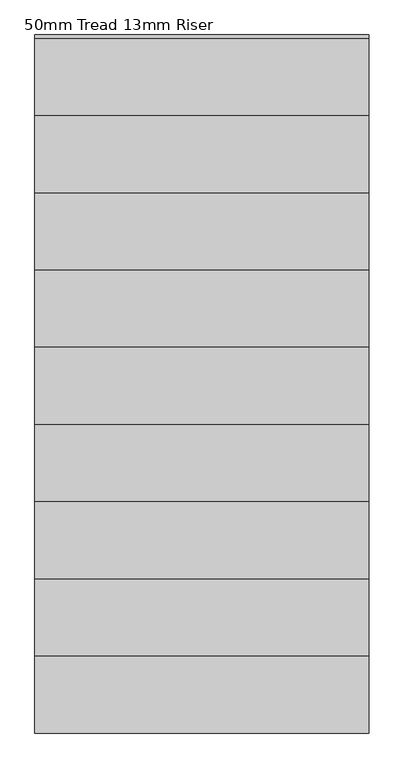
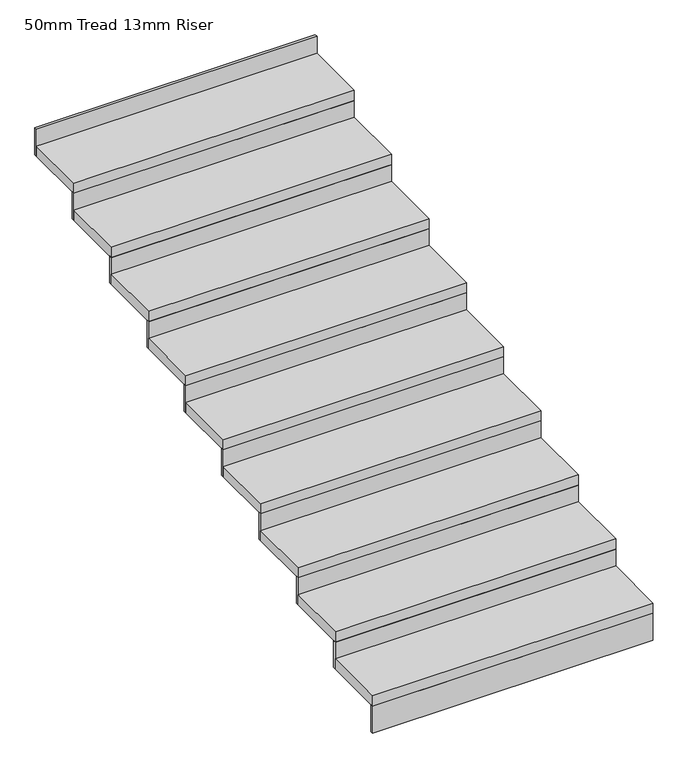
"""IFC4 building model written with IfcOpenShell, lengths in millimetres: stair flight geometry, 50mm Tread 13mm Riser."""

from ifc_helpers import new_model, si_unit, frame, origin, place, context, project, spatial, polyline, outline, extrude, source, transform, mapped, element, save


def stair_flight_50mm_tread_13mm_riser_1c1921b2(model_context):
    return source(origin(), model_context, "Body", "SweptSolid", [
        extrude(outline(polyline([(-13276.101437, -1585.8427081), (-13276.101437, -1598.3427081), (-14576.101437, -1598.3427081), (-14576.101437, -1585.8427081), (-13276.101437, -1585.8427081)])), frame((0.0, 0.0, 4270.0), z_axis=(0.0, 0.0, 1.0), x_axis=(1.0, 0.0, 0.0)), (0.0, 0.0, 1.0), 132.0),
        extrude(outline(polyline([(-14576.101437, -1298.3427081), (-13276.101437, -1298.3427081), (-13276.101437, -1598.3427081), (-14576.101437, -1598.3427081), (-14576.101437, -1298.3427081)])), frame((0.0, 0.0, 4402.0), z_axis=(0.0, 0.0, 1.0), x_axis=(1.0, 0.0, 0.0)), (0.0, 0.0, 1.0), 50.0),
        extrude(outline(polyline([(-13276.101437, -1285.8427081), (-13276.101437, -1298.3427081), (-14576.101437, -1298.3427081), (-14576.101437, -1285.8427081), (-13276.101437, -1285.8427081)])), frame((0.0, 0.0, 4402.0), z_axis=(0.0, 0.0, 1.0), x_axis=(1.0, 0.0, 0.0)), (0.0, 0.0, 1.0), 132.0),
        extrude(outline(polyline([(-14576.101437, -998.3427081), (-13276.101437, -998.3427081), (-13276.101437, -1298.3427081), (-14576.101437, -1298.3427081), (-14576.101437, -998.3427081)])), frame((0.0, 0.0, 4534.0), z_axis=(0.0, 0.0, 1.0), x_axis=(1.0, 0.0, 0.0)), (0.0, 0.0, 1.0), 50.0),
        extrude(outline(polyline([(-13276.101437, -985.8427081), (-13276.101437, -998.3427081), (-14576.101437, -998.3427081), (-14576.101437, -985.8427081), (-13276.101437, -985.8427081)])), frame((0.0, 0.0, 4534.0), z_axis=(0.0, 0.0, 1.0), x_axis=(1.0, 0.0, 0.0)), (0.0, 0.0, 1.0), 132.0),
        extrude(outline(polyline([(-14576.101437, -698.3427081), (-13276.101437, -698.3427081), (-13276.101437, -998.3427081), (-14576.101437, -998.3427081), (-14576.101437, -698.3427081)])), frame((0.0, 0.0, 4666.0), z_axis=(0.0, 0.0, 1.0), x_axis=(1.0, 0.0, 0.0)), (0.0, 0.0, 1.0), 50.0),
        extrude(outline(polyline([(-13276.101437, -685.8427081), (-13276.101437, -698.3427081), (-14576.101437, -698.3427081), (-14576.101437, -685.8427081), (-13276.101437, -685.8427081)])), frame((0.0, 0.0, 4666.0), z_axis=(0.0, 0.0, 1.0), x_axis=(1.0, 0.0, 0.0)), (0.0, 0.0, 1.0), 132.0),
        extrude(outline(polyline([(-14576.101437, -398.3427081), (-13276.101437, -398.3427081), (-13276.101437, -698.3427081), (-14576.101437, -698.3427081), (-14576.101437, -398.3427081)])), frame((0.0, 0.0, 4798.0), z_axis=(0.0, 0.0, 1.0), x_axis=(1.0, 0.0, 0.0)), (0.0, 0.0, 1.0), 50.0),
        extrude(outline(polyline([(-13276.101437, -385.8427081), (-13276.101437, -398.3427081), (-14576.101437, -398.3427081), (-14576.101437, -385.8427081), (-13276.101437, -385.8427081)])), frame((0.0, 0.0, 4798.0), z_axis=(0.0, 0.0, 1.0), x_axis=(1.0, 0.0, 0.0)), (0.0, 0.0, 1.0), 132.0),
        extrude(outline(polyline([(-14576.101437, -98.3427081), (-13276.101437, -98.3427081), (-13276.101437, -398.3427081), (-14576.101437, -398.3427081), (-14576.101437, -98.3427081)])), frame((0.0, 0.0, 4930.0), z_axis=(0.0, 0.0, 1.0), x_axis=(1.0, 0.0, 0.0)), (0.0, 0.0, 1.0), 50.0),
        extrude(outline(polyline([(-13276.101437, -85.8427081), (-13276.101437, -98.3427081), (-14576.101437, -98.3427081), (-14576.101437, -85.8427081), (-13276.101437, -85.8427081)])), frame((0.0, 0.0, 4930.0), z_axis=(0.0, 0.0, 1.0), x_axis=(1.0, 0.0, 0.0)), (0.0, 0.0, 1.0), 132.0),
        extrude(outline(polyline([(-14576.101437, 201.6572919), (-13276.101437, 201.6572919), (-13276.101437, -98.3427081), (-14576.101437, -98.3427081), (-14576.101437, 201.6572919)])), frame((0.0, 0.0, 5062.0), z_axis=(0.0, 0.0, 1.0), x_axis=(1.0, 0.0, 0.0)), (0.0, 0.0, 1.0), 50.0),
        extrude(outline(polyline([(-13276.101437, 214.1572919), (-13276.101437, 201.6572919), (-14576.101437, 201.6572919), (-14576.101437, 214.1572919), (-13276.101437, 214.1572919)])), frame((0.0, 0.0, 5062.0), z_axis=(0.0, 0.0, 1.0), x_axis=(1.0, 0.0, 0.0)), (0.0, 0.0, 1.0), 132.0),
        extrude(outline(polyline([(-14576.101437, 501.6572919), (-13276.101437, 501.6572919), (-13276.101437, 201.6572919), (-14576.101437, 201.6572919), (-14576.101437, 501.6572919)])), frame((0.0, 0.0, 5194.0), z_axis=(0.0, 0.0, 1.0), x_axis=(1.0, 0.0, 0.0)), (0.0, 0.0, 1.0), 50.0),
        extrude(outline(polyline([(-13276.101437, 514.1572919), (-13276.101437, 501.6572919), (-14576.101437, 501.6572919), (-14576.101437, 514.1572919), (-13276.101437, 514.1572919)])), frame((0.0, 0.0, 5194.0), z_axis=(0.0, 0.0, 1.0), x_axis=(1.0, 0.0, 0.0)), (0.0, 0.0, 1.0), 132.0),
        extrude(outline(polyline([(-14576.101437, 801.6572919), (-13276.101437, 801.6572919), (-13276.101437, 501.6572919), (-14576.101437, 501.6572919), (-14576.101437, 801.6572919)])), frame((0.0, 0.0, 5326.0), z_axis=(0.0, 0.0, 1.0), x_axis=(1.0, 0.0, 0.0)), (0.0, 0.0, 1.0), 50.0),
        extrude(outline(polyline([(-13276.101437, 814.1572919), (-13276.101437, 801.6572919), (-14576.101437, 801.6572919), (-14576.101437, 814.1572919), (-13276.101437, 814.1572919)])), frame((0.0, 0.0, 5326.0), z_axis=(0.0, 0.0, 1.0), x_axis=(1.0, 0.0, 0.0)), (0.0, 0.0, 1.0), 132.0),
        extrude(outline(polyline([(-13276.101437, 1114.1572919), (-13276.101437, 1101.6572919), (-14576.101437, 1101.6572919), (-14576.101437, 1114.1572919), (-13276.101437, 1114.1572919)])), frame((0.0, 0.0, 5458.0), z_axis=(0.0, 0.0, 1.0), x_axis=(1.0, 0.0, 0.0)), (0.0, 0.0, 1.0), 132.0),
        extrude(outline(polyline([(-14576.101437, 1101.6572919), (-13276.101437, 1101.6572919), (-13276.101437, 801.6572919), (-14576.101437, 801.6572919), (-14576.101437, 1101.6572919)])), frame((0.0, 0.0, 5458.0), z_axis=(0.0, 0.0, 1.0), x_axis=(1.0, 0.0, 0.0)), (0.0, 0.0, 1.0), 50.0),
    ])


if __name__ == "__main__":
    model = new_model("IFC4")
    model_context = context("Model", 3, world=origin())
    ifc_project = project(units=[si_unit("LENGTHUNIT", "METRE", prefix="MILLI")], contexts=[model_context])
    site = spatial("IfcSite", under=ifc_project)
    building = spatial("IfcBuilding", under=site)
    placement = place(None, origin())
    stair_flight_50mm_tread_13mm_riser_shape = stair_flight_50mm_tread_13mm_riser_1c1921b2(model_context)
    element("IfcStairFlight", 1, ObjectType="50mm Tread 13mm Riser", at=placement, inside=building, context=model_context, shape_type="MappedRepresentation", body=[
        mapped(stair_flight_50mm_tread_13mm_riser_shape, transform((0.0, 0.0, 0.0), x_axis=(1.0, 0.0, 0.0), y_axis=(0.0, 1.0, 0.0), z_axis=(0.0, 0.0, 1.0))),
    ])
    save(model, "model.ifc")
